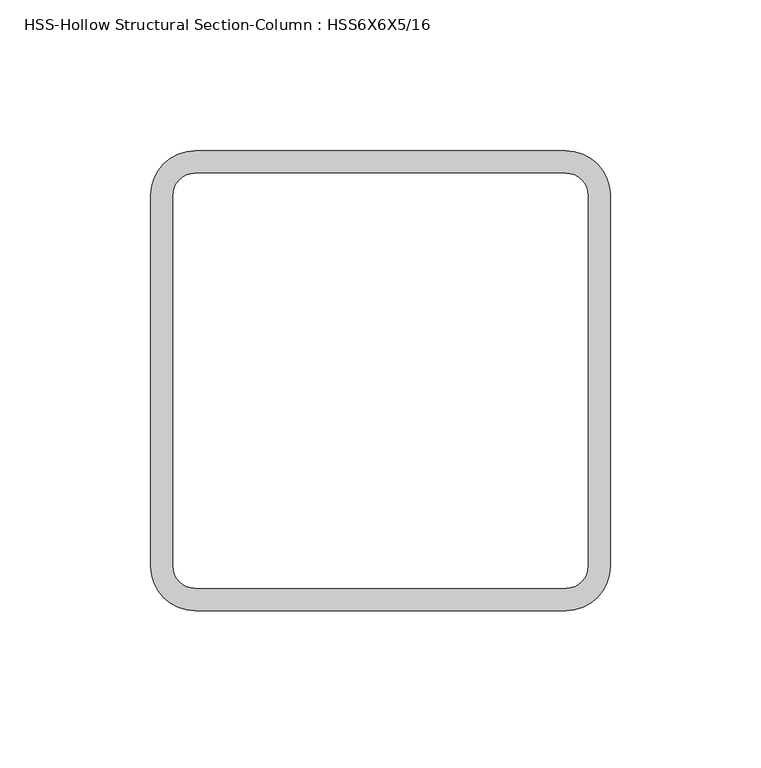
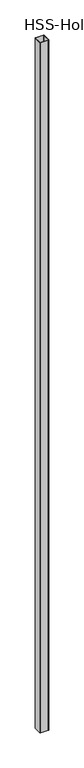
"""IFC4 building model written with IfcOpenShell, lengths in millimetres: column geometry, HSS-Hollow Structural Section-Column : HSS6X6X5/16."""

from ifc_helpers import new_model, si_unit, point, frame, frame_2d, origin, place, context, project, spatial, polyline, circle_curve, trimmed, segment, composite_curve, outline, extrude, source, transform, mapped, element, save


def hss_hollow_structural_section_column_hss6x6x5_16_437795de(model_context):
    return source(origin(), model_context, "Body", "SweptSolid", [
        extrude(outline(composite_curve([segment(trimmed(circle_curve(frame_2d((61.4172, 61.4172)), 14.7828), [point((61.4172, 76.2))], [point((76.2, 61.4172))], False, "CARTESIAN"), True, "CONTINUOUS"), segment(polyline([(76.2, 61.4172), (76.2, -61.4172)]), True, "CONTINUOUS"), segment(trimmed(circle_curve(frame_2d((61.4172, -61.4172)), 14.7828), [point((76.2, -61.4172))], [point((61.4172, -76.2))], False, "CARTESIAN"), True, "CONTINUOUS"), segment(polyline([(61.4172, -76.2), (-61.4172, -76.2)]), True, "CONTINUOUS"), segment(trimmed(circle_curve(frame_2d((-61.4172, -61.4172)), 14.7828), [point((-61.4172, -76.2))], [point((-76.2, -61.4172))], False, "CARTESIAN"), True, "CONTINUOUS"), segment(polyline([(-76.2, -61.4172), (-76.2, 61.4172)]), True, "CONTINUOUS"), segment(trimmed(circle_curve(frame_2d((-61.4172, 61.4172)), 14.7828), [point((-76.2, 61.4172))], [point((-61.4172, 76.2))], False, "CARTESIAN"), True, "CONTINUOUS"), segment(polyline([(-61.4172, 76.2), (61.4172, 76.2)]), True, "CONTINUOUS")], self_intersect=False), holes=[composite_curve([segment(polyline([(61.4172, 68.8086), (-61.4172, 68.8086)]), True, "CONTINUOUS"), segment(trimmed(circle_curve(frame_2d((-61.4172, 61.4172)), 7.3914), [point((-61.4172, 68.8086))], [point((-68.8086, 61.4172))], True, "CARTESIAN"), True, "CONTINUOUS"), segment(polyline([(-68.8086, 61.4172), (-68.8086, -61.4172)]), True, "CONTINUOUS"), segment(trimmed(circle_curve(frame_2d((-61.4172, -61.4172)), 7.3914), [point((-68.8086, -61.4172))], [point((-61.4172, -68.8086))], True, "CARTESIAN"), True, "CONTINUOUS"), segment(polyline([(-61.4172, -68.8086), (61.4172, -68.8086)]), True, "CONTINUOUS"), segment(trimmed(circle_curve(frame_2d((61.4172, -61.4172)), 7.3914), [point((61.4172, -68.8086))], [point((68.8086, -61.4172))], True, "CARTESIAN"), True, "CONTINUOUS"), segment(polyline([(68.8086, -61.4172), (68.8086, 61.4172)]), True, "CONTINUOUS"), segment(trimmed(circle_curve(frame_2d((61.4172, 61.4172)), 7.3914), [point((68.8086, 61.4172))], [point((61.4172, 68.8086))], True, "CARTESIAN"), True, "CONTINUOUS")], self_intersect=False)]), frame((0.0, 0.0, 12566.65), z_axis=(0.0, 0.0, 1.0), x_axis=(1.0, 0.0, 0.0)), (0.0, 0.0, 1.0), 12376.15),
    ])


if __name__ == "__main__":
    model = new_model("IFC4")
    model_context = context("Model", 3, world=origin())
    ifc_project = project(units=[si_unit("LENGTHUNIT", "METRE", prefix="MILLI")], contexts=[model_context])
    site = spatial("IfcSite", under=ifc_project)
    building = spatial("IfcBuilding", under=site)
    placement = place(None, origin())
    hss_hollow_structural_section_column_hss6x6x5_16_shape = hss_hollow_structural_section_column_hss6x6x5_16_437795de(model_context)
    element("IfcColumn", 1, ObjectType="HSS-Hollow Structural Section-Column : HSS6X6X5/16", at=placement, inside=building, context=model_context, shape_type="MappedRepresentation", body=[
        mapped(hss_hollow_structural_section_column_hss6x6x5_16_shape, transform((0.0, 0.0, 0.0), x_axis=(1.0, 0.0, 0.0), y_axis=(0.0, 1.0, 0.0), z_axis=(0.0, 0.0, 1.0))),
    ])
    save(model, "model.ifc")

# Revit data of these elements
# Type "HSS-Hollow Structural Section-Column : HSS6X6X5/16"
#   Assembly Code = "B10"
#   Shape = "Square"
#   W = 23.3
#   Ht = 0' - 6"
#   b = 0' - 6"
#   kr = 0' - 0.582"
#   t = 0' - 0.291"
#   A = 0.0446528 SF
#   Structural Material [instance default] = Steel ASTM A500, Grade B, Rectangular and Square
# Element 1 (IfcColumn, "HSS-Hollow Structural Section-Column : HSS6X6X5/16")
#   Materials on its faces: "Steel ASTM A500, Grade B, Rectangular and Square"
# Materials
#   "Steel ASTM A500, Grade B, Rectangular and Square": class "Metal", colour RGB 199 199 199, transparency 0, Description = "Carbon steel", Cost = 0
